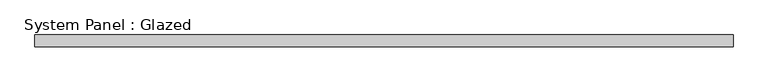
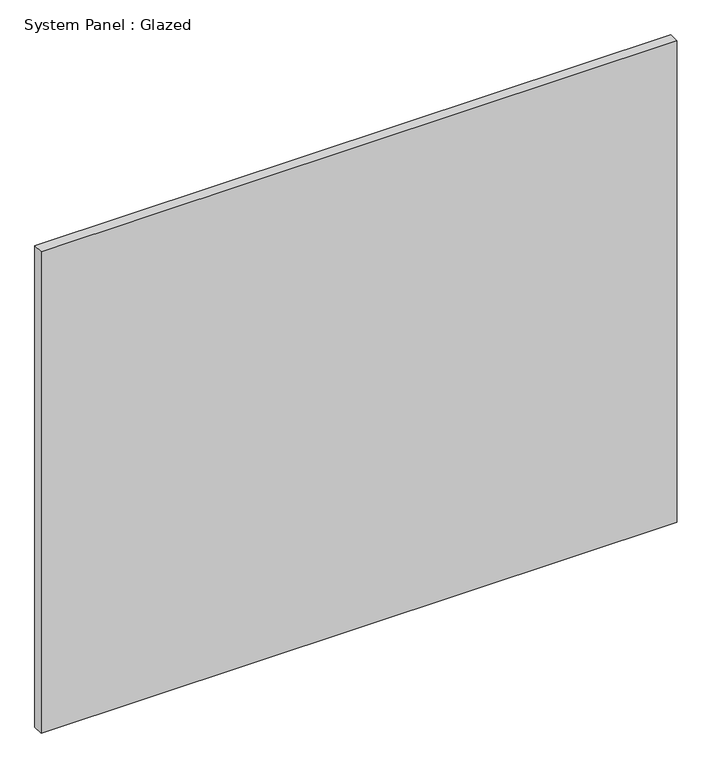
"""IFC4 building model written with IfcOpenShell, lengths in millimetres: plate geometry, System Panel : Glazed."""

from ifc_helpers import new_model, si_unit, origin, origin_with_axes, place, context, project, spatial, polyline, outline, extrude, source, transform, mapped, element, save


def system_panel_glazed_14200f5a(model_context):
    return source(origin(), model_context, "Body", "SweptSolid", [
        extrude(outline(polyline([(762.0, 19.05), (-762.0, 19.05), (-762.0, 44.45), (762.0, 44.45), (762.0, 19.05)])), origin_with_axes(), (0.0, 0.0, 1.0), 1219.2),
    ])


if __name__ == "__main__":
    model = new_model("IFC4")
    model_context = context("Model", 3, world=origin())
    ifc_project = project(units=[si_unit("LENGTHUNIT", "METRE", prefix="MILLI")], contexts=[model_context])
    site = spatial("IfcSite", under=ifc_project)
    building = spatial("IfcBuilding", under=site)
    placement = place(None, origin())
    system_panel_glazed_shape = system_panel_glazed_14200f5a(model_context)
    element("IfcPlate", 1, ObjectType="System Panel : Glazed", at=placement, inside=building, context=model_context, shape_type="MappedRepresentation", body=[
        mapped(system_panel_glazed_shape, transform((0.0, 0.0, 0.0), x_axis=(1.0, 0.0, 0.0), y_axis=(0.0, 1.0, 0.0), z_axis=(0.0, 0.0, 1.0))),
    ])
    save(model, "model.ifc")

# Revit data of these elements
# Element 1 (IfcPlate, "System Panel : Glazed")
#   Materials on its faces: "Glass"
# Materials
#   "Glass": class "Glass", colour RGB 0 128 192, transparency 0.75
